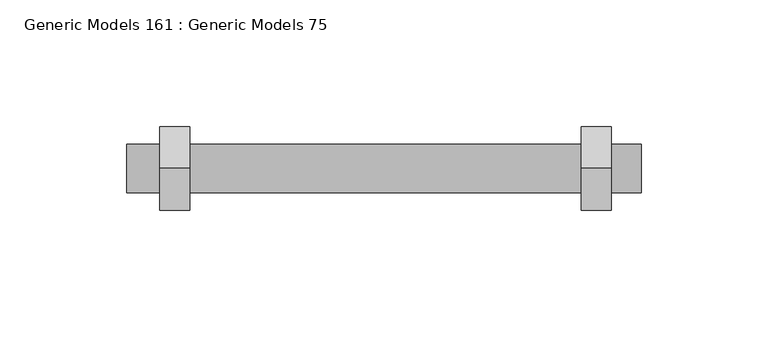
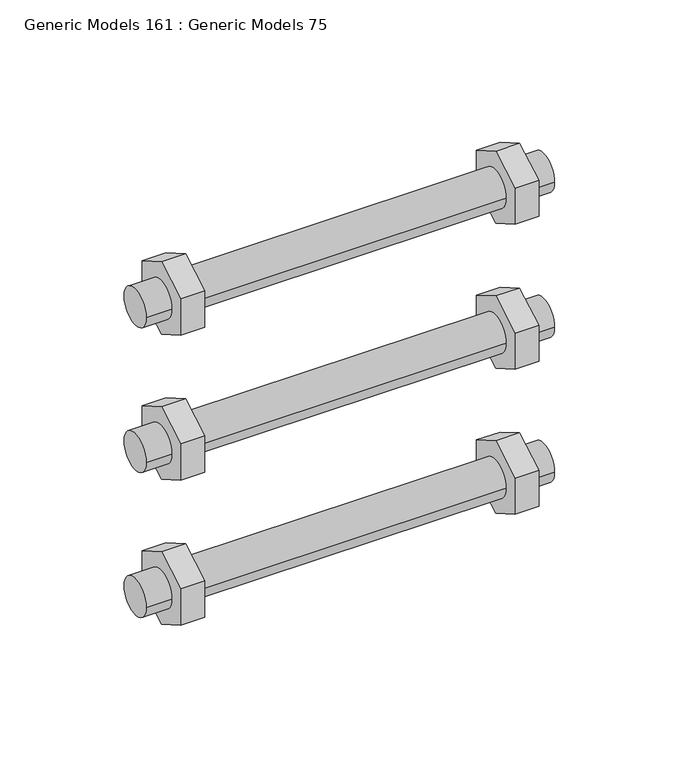
"""IFC4 building model written with IfcOpenShell, lengths in millimetres: proxy geometry, Generic Models 161 : Generic Models 75."""

from ifc_helpers import new_model, si_unit, point, frame, frame_2d, origin, place, context, project, spatial, polyline, circle_curve, trimmed, segment, composite_curve, outline, extrude, source, transform, mapped, element, save


def generic_models_161_generic_models_75_eba7e698(model_context):
    return source(origin(), model_context, "Body", "SweptSolid", [
        extrude(outline(polyline([(36529.8292603, 271852.097122), (36546.3270442, 271861.622122), (36562.8248281, 271852.097122), (36562.8248281, 271833.047122), (36546.3270442, 271823.522122), (36529.8292603, 271833.047122), (36529.8292603, 271852.097122)])), frame((31918.2596032, 0.0, 0.0), z_axis=(1.0, 0.0, 0.0), x_axis=(0.0, 1.0, 0.0)), (0.0, 0.0, 1.0), 11.90625),
        extrude(outline(polyline([(36529.8292603, 271775.897122), (36546.3270442, 271785.422122), (36562.8248281, 271775.897122), (36562.8248281, 271756.847122), (36546.3270442, 271747.322122), (36529.8292603, 271756.847122), (36529.8292603, 271775.897122)])), frame((31918.2596032, 0.0, 0.0), z_axis=(1.0, 0.0, 0.0), x_axis=(0.0, 1.0, 0.0)), (0.0, 0.0, 1.0), 11.90625),
        extrude(outline(polyline([(36529.8292603, 271699.697122), (36546.3270442, 271709.222122), (36562.8248281, 271699.697122), (36562.8248281, 271680.647122), (36546.3270442, 271671.122122), (36529.8292603, 271680.647122), (36529.8292603, 271699.697122)])), frame((31918.2596032, 0.0, 0.0), z_axis=(1.0, 0.0, 0.0), x_axis=(0.0, 1.0, 0.0)), (0.0, 0.0, 1.0), 11.90625),
        extrude(outline(polyline([(36529.8292603, 271852.097122), (36546.3270442, 271861.622122), (36562.8248281, 271852.097122), (36562.8248281, 271833.047122), (36546.3270442, 271823.522122), (36529.8292603, 271833.047122), (36529.8292603, 271852.097122)])), frame((31751.9689782, 0.0, 0.0), z_axis=(1.0, 0.0, 0.0), x_axis=(0.0, 1.0, 0.0)), (0.0, 0.0, 1.0), 11.90625),
        extrude(outline(polyline([(36529.8292603, 271775.897122), (36546.3270442, 271785.422122), (36562.8248281, 271775.897122), (36562.8248281, 271756.847122), (36546.3270442, 271747.322122), (36529.8292603, 271756.847122), (36529.8292603, 271775.897122)])), frame((31751.9689782, 0.0, 0.0), z_axis=(1.0, 0.0, 0.0), x_axis=(0.0, 1.0, 0.0)), (0.0, 0.0, 1.0), 11.90625),
        extrude(outline(polyline([(36529.8292603, 271699.697122), (36546.3270442, 271709.222122), (36562.8248281, 271699.697122), (36562.8248281, 271680.647122), (36546.3270442, 271671.122122), (36529.8292603, 271680.647122), (36529.8292603, 271699.697122)])), frame((31751.9689782, 0.0, 0.0), z_axis=(1.0, 0.0, 0.0), x_axis=(0.0, 1.0, 0.0)), (0.0, 0.0, 1.0), 11.90625),
        extrude(outline(composite_curve([segment(trimmed(circle_curve(frame_2d((36546.3270442, 271766.372122)), 9.525), [point((36555.8520442, 271766.372122))], [point((36536.8020442, 271766.372122))], False, "CARTESIAN"), True, "CONTINUOUS"), segment(trimmed(circle_curve(frame_2d((36546.3270442, 271766.372122)), 9.525), [point((36536.8020442, 271766.372122))], [point((36555.8520442, 271766.372122))], False, "CARTESIAN"), True, "CONTINUOUS")], self_intersect=False)), frame((31738.8721032, 0.0, 0.0), z_axis=(1.0, 0.0, 0.0), x_axis=(0.0, 1.0, 0.0)), (0.0, 0.0, 1.0), 203.2),
        extrude(outline(composite_curve([segment(trimmed(circle_curve(frame_2d((36546.3270442, 271690.172122)), 9.525), [point((36555.8520442, 271690.172122))], [point((36536.8020442, 271690.172122))], False, "CARTESIAN"), True, "CONTINUOUS"), segment(trimmed(circle_curve(frame_2d((36546.3270442, 271690.172122)), 9.525), [point((36536.8020442, 271690.172122))], [point((36555.8520442, 271690.172122))], False, "CARTESIAN"), True, "CONTINUOUS")], self_intersect=False)), frame((31738.8721032, 0.0, 0.0), z_axis=(1.0, 0.0, 0.0), x_axis=(0.0, 1.0, 0.0)), (0.0, 0.0, 1.0), 203.2),
        extrude(outline(composite_curve([segment(trimmed(circle_curve(frame_2d((36546.3270442, 271842.572122)), 9.525), [point((36555.8520442, 271842.572122))], [point((36536.8020442, 271842.572122))], False, "CARTESIAN"), True, "CONTINUOUS"), segment(trimmed(circle_curve(frame_2d((36546.3270442, 271842.572122)), 9.525), [point((36536.8020442, 271842.572122))], [point((36555.8520442, 271842.572122))], False, "CARTESIAN"), True, "CONTINUOUS")], self_intersect=False)), frame((31738.8721032, 0.0, 0.0), z_axis=(1.0, 0.0, 0.0), x_axis=(0.0, 1.0, 0.0)), (0.0, 0.0, 1.0), 203.2),
    ])


if __name__ == "__main__":
    model = new_model("IFC4")
    model_context = context("Model", 3, world=origin())
    ifc_project = project(units=[si_unit("LENGTHUNIT", "METRE", prefix="MILLI")], contexts=[model_context])
    site = spatial("IfcSite", under=ifc_project)
    building = spatial("IfcBuilding", under=site)
    placement = place(None, origin())
    generic_models_161_generic_models_75_shape = generic_models_161_generic_models_75_eba7e698(model_context)
    element("IfcBuildingElementProxy", 1, Name="Generic Models 161 : Generic Models 75", ObjectType="Generic Models 161 : Generic Models 75", at=placement, inside=building, context=model_context, shape_type="MappedRepresentation", body=[
        mapped(generic_models_161_generic_models_75_shape, transform((0.0, 0.0, 0.0), x_axis=(1.0, 0.0, 0.0), y_axis=(0.0, 1.0, 0.0), z_axis=(0.0, 0.0, 1.0))),
    ])
    save(model, "model.ifc")
